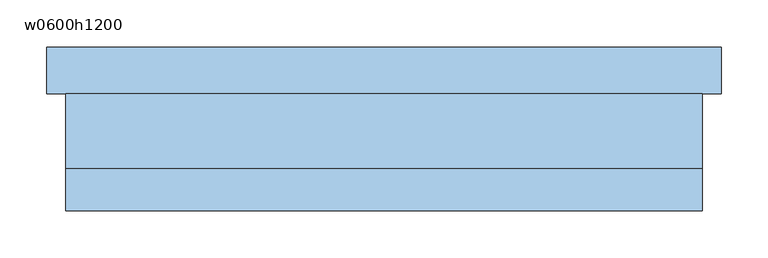
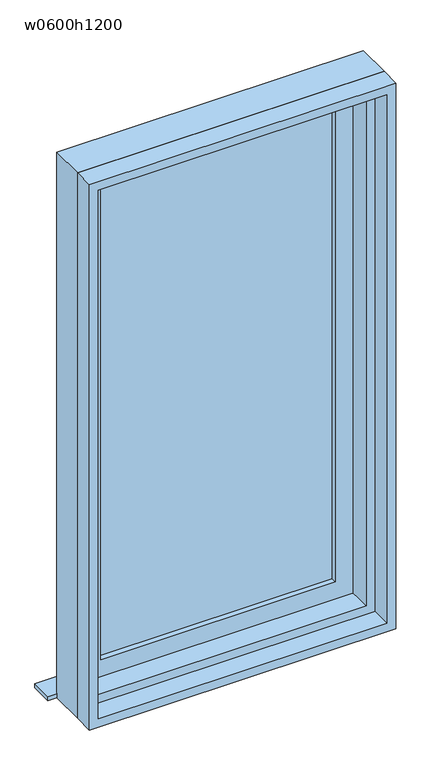
"""IFC4 building model written with IfcOpenShell, lengths in millimetres: window geometry, 縦すべり窓 : w0600h1200."""

from ifc_helpers import new_model, si_unit, frame, origin, place, context, project, spatial, polyline, outline, extrude, source, transform, mapped, element, save


def w0600h1200_d3eda8cc(model_context):
    return source(origin(), model_context, "Body", "SweptSolid", [
        extrude(outline(polyline([(260.0, 22.5), (-260.0, 22.5), (-260.0, 27.5), (260.0, 27.5), (260.0, 22.5)])), frame((0.0, 0.0, 840.0), z_axis=(0.0, 0.0, 1.0), x_axis=(1.0, 0.0, 0.0)), (0.0, 0.0, 1.0), 1120.0),
        extrude(outline(polyline([(2000.0, 300.0), (2000.0, -300.0), (800.0, -300.0), (800.0, 300.0), (2000.0, 300.0)]), holes=[polyline([(1960.0, -260.0), (1960.0, 260.0), (840.0, 260.0), (840.0, -260.0), (1960.0, -260.0)])]), frame((0.0, 10.0, 0.0), z_axis=(0.0, 1.0, 0.0), x_axis=(0.0, 0.0, 1.0)), (0.0, 0.0, 1.0), 30.0),
        extrude(outline(polyline([(360.0, 90.0), (360.0, 40.0), (-360.0, 40.0), (-360.0, 90.0), (360.0, 90.0)])), frame((0.0, 0.0, 760.0), z_axis=(0.0, 0.0, 1.0), x_axis=(1.0, 0.0, 0.0)), (0.0, 0.0, 1.0), 10.0),
        extrude(outline(polyline([(2040.0, 340.0), (2040.0, -340.0), (760.0, -340.0), (760.0, 340.0), (2040.0, 340.0)]), holes=[polyline([(780.0, -320.0), (2020.0, -320.0), (2020.0, 320.0), (780.0, 320.0), (780.0, -320.0)])]), frame((0.0, -85.0, 0.0), z_axis=(0.0, 1.0, 0.0), x_axis=(0.0, 0.0, 1.0)), (0.0, 0.0, 1.0), 45.0),
        extrude(outline(polyline([(2040.0, -340.0), (760.0, -340.0), (760.0, 340.0), (2040.0, 340.0), (2040.0, -340.0)]), holes=[polyline([(2000.0, 300.0), (800.0, 300.0), (800.0, -300.0), (2000.0, -300.0), (2000.0, 300.0)])]), frame((0.0, -40.0, 0.0), z_axis=(0.0, 1.0, 0.0), x_axis=(0.0, 0.0, 1.0)), (0.0, 0.0, 1.0), 80.0),
    ])


if __name__ == "__main__":
    model = new_model("IFC4")
    model_context = context("Model", 3, world=origin())
    ifc_project = project(units=[si_unit("LENGTHUNIT", "METRE", prefix="MILLI")], contexts=[model_context])
    site = spatial("IfcSite", under=ifc_project)
    building = spatial("IfcBuilding", under=site)
    placement = place(None, origin())
    w0600h1200_shape = w0600h1200_d3eda8cc(model_context)
    element("IfcWindow", 1, ObjectType="縦すべり窓 : w0600h1200", at=placement, inside=building, context=model_context, shape_type="MappedRepresentation", body=[
        mapped(w0600h1200_shape, transform((0.0, 0.0, 0.0), x_axis=(1.0, 0.0, 0.0), y_axis=(0.0, 1.0, 0.0), z_axis=(0.0, 0.0, 1.0))),
    ])
    save(model, "model.ifc")

# Revit data of these elements
# Type "縦すべり窓 : w0600h1200"
#   Construction Type Id = "GSP4R"
#   Analytic Construction = "1/8 インチ ピルキントン一重ガラス"
#   Type Mark = "86"
#   Operation = "シングルパネル"
#   Keynote = "08520.S3"
#   Visual Light Transmittance = 0.9
#   Solar Heat Gain Coefficient = 0.86
#   Heat Transfer Coefficient (U) = 6.7069 W/(m²·K)
#   Height = 1200 mm
#   既定の腰高 = 800 mm
#   Width = 600 mm
#   額縁見附 = 20 mm
#   額縁ちり = 10 mm
#   サッシ見附 = 40 mm
#   サッシの幅 = 80 mm
#   サッシ額縁 [instance default] = none
#   サッシ本体 [instance default] = none
#   サッシガラス [instance default] = ガラス - 透明
#   Wall Closure = (empty or 0)
#   Type Comments = ""
#   Assembly Code = ""
# Element 1 (IfcWindow, "縦すべり窓 : w0600h1200")
#   Materials on its faces: "ガラス - 透明"
# Materials
#   "ガラス - 透明": class "ガラス", colour RGB 0 128 192, transparency 0.9, Cost = 0
